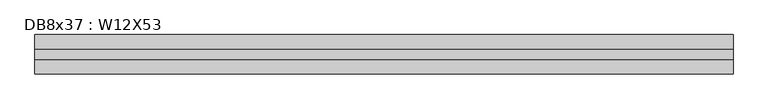
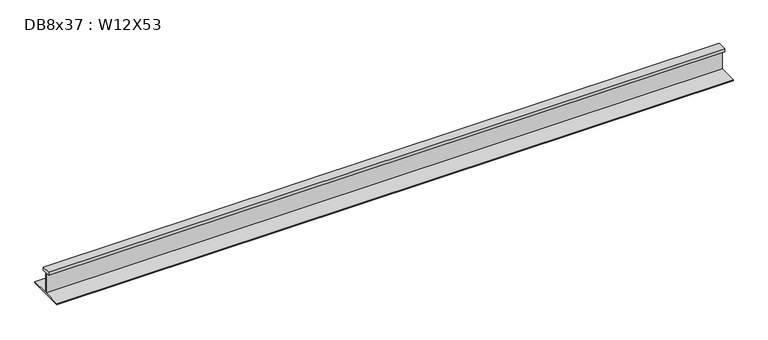
"""IFC4 building model written with IfcOpenShell, lengths in millimetres: beam geometry, DB8x37 : W12X53."""

from ifc_helpers import new_model, si_unit, frame, origin, place, context, project, spatial, polyline, outline, extrude, source, transform, mapped, element, save


def db8x37_w12x53_736502ec(model_context):
    return source(origin(), model_context, "Body", "SweptSolid", [
        extrude(outline(polyline([(38.1, 145.415), (38.1, 120.015), (2.921, 120.015), (2.921, -48.4505), (152.4, -48.4505), (152.4, -58.1025), (-152.4, -58.1025), (-152.4, -48.4505), (-2.921, -48.4505), (-2.921, 120.015), (-38.1, 120.015), (-38.1, 145.415), (38.1, 145.415)])), frame((-2703.83, 0.0, 0.0), z_axis=(1.0, 0.0, 0.0), x_axis=(0.0, 1.0, 0.0)), (0.0, 0.0, 1.0), 5407.66),
    ])


if __name__ == "__main__":
    model = new_model("IFC4")
    model_context = context("Model", 3, world=origin())
    ifc_project = project(units=[si_unit("LENGTHUNIT", "METRE", prefix="MILLI")], contexts=[model_context])
    site = spatial("IfcSite", under=ifc_project)
    building = spatial("IfcBuilding", under=site)
    placement = place(None, origin())
    db8x37_w12x53_shape = db8x37_w12x53_736502ec(model_context)
    element("IfcBeam", 1, ObjectType="DB8x37 : W12X53", at=placement, inside=building, context=model_context, shape_type="MappedRepresentation", body=[
        mapped(db8x37_w12x53_shape, transform((0.0, 0.0, 0.0), x_axis=(1.0, 0.0, 0.0), y_axis=(0.0, 1.0, 0.0), z_axis=(0.0, 0.0, 1.0))),
    ])
    save(model, "model.ifc")

# Revit data of these elements
# Type "DB8x37 : W12X53"
#   Assembly Code = "B10"
#   W = 53
#   Length [instance default] = 5' - 0"
#   bf = 0' - 10"
#   d = 1' - 0.1"
#   k = 0' - 1 3/8"
#   k2 = 0' - 0.8"
#   tf = 0' - 0.575"
#   tw = 0' - 0.345"
#   A = 0.108333 SF
#   Structural Material [instance default] = Steel ASTM A992
# Element 1 (IfcBeam, "DB8x37 : W12X53")
#   Materials on its faces: "Steel ASTM A992"
# Materials
#   "Steel ASTM A992": class "Metal", colour RGB 199 199 199, transparency 0, Description = "Structural steel 50ksi", Cost = 0
